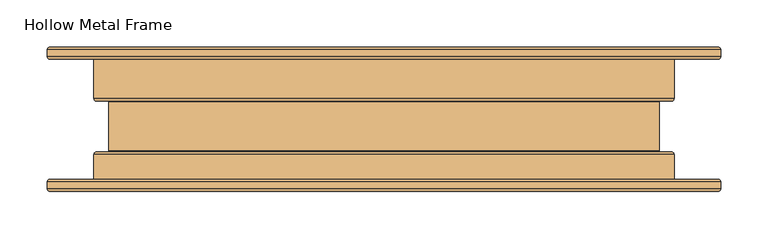
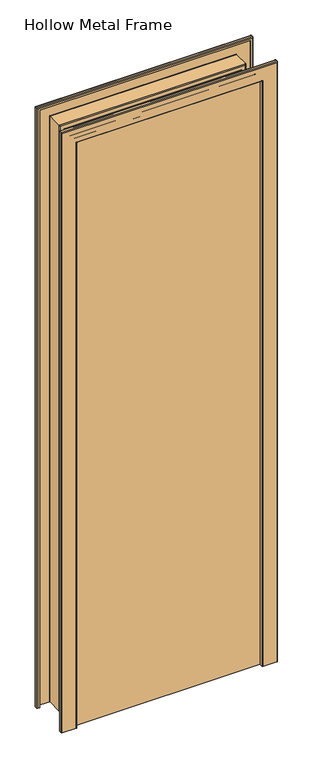
"""IFC4 building model written with IfcOpenShell, lengths in millimetres: door geometry, Hollow Metal Frame."""

from ifc_helpers import new_model, si_unit, frame, origin, origin_with_axes, place, context, project, spatial, polyline, circle_curve, ellipse_curve, outline, extrude, source, transform, mapped, element, save
from ifc_brep_helpers import plane_surface, cylinder_surface, revolved_surface, advanced_brep


def hollow_metal_frame_48c6d259(model_context):
    return source(origin(), model_context, "Body", "SolidModel", [
        advanced_brep(
        [(-353.02825, 63.5635, 0.0), (-355.6, 66.13525, 0.0), (-355.6, 73.66, 0.0), (-353.02825, 76.23175, 0.0), (-307.37175, 76.23175, 0.0), (-304.8, 73.66, 0.0), (-304.8, 21.68525, 0.0), (-303.784, 20.66925, 0.0), (-291.49675, 20.66925, 0.0), (-288.925, 18.0975, 0.0), (-288.925, -33.6931, 0.0), (-291.49675, -36.26485, 0.0), (-303.784, -36.26485, 0.0), (-304.8, -37.28085, 0.0), (-304.8, -73.5965, 0.0), (-307.37175, -76.16825, 0.0), (-353.02825, -76.16825, 0.0), (-355.6, -73.5965, 0.0), (-355.6, -66.07175, 0.0), (-353.02825, -63.5, 0.0), (-347.6625, -63.5, 0.0), (-347.6625, -65.05575, 0.0), (-353.02825, -65.05575, 0.0), (-354.04425, -66.07175, 0.0), (-354.04425, -73.5965, 0.0), (-353.02825, -74.6125, 0.0), (-307.37175, -74.6125, 0.0), (-306.35575, -73.5965, 0.0), (-306.35575, -37.28085, 0.0), (-303.784, -34.7091, 0.0), (-291.49675, -34.7091, 0.0), (-290.48075, -33.6931, 0.0), (-290.48075, 18.0975, 0.0), (-291.49675, 19.1135, 0.0), (-303.784, 19.1135, 0.0), (-306.35575, 21.68525, 0.0), (-306.35575, 73.66, 0.0), (-307.37175, 74.676, 0.0), (-353.02825, 74.676, 0.0), (-354.04425, 73.66, 0.0), (-354.04425, 66.13525, 0.0), (-353.02825, 65.11925, 0.0), (-347.6625, 65.11925, 0.0), (-347.6625, 63.5635, 0.0), (-353.02825, 63.5635, 2080.2282501), (-355.6, 66.13525, 2082.8000001), (-355.6, 73.66, 2082.8000001), (-353.02825, 76.23175, 2080.2282501), (353.02825, 76.23175, 2080.2282501), (353.02825, 76.23175, 0.0), (307.37175, 76.23175, 0.0), (307.37175, 76.23175, 2034.5717501), (-307.37175, 76.23175, 2034.5717501), (-304.8, 73.66, 2032.0000001), (-304.8, 21.68525, 2032.0000001), (-303.784, 20.66925, 2030.9840001), (303.784, 20.66925, 2030.9840001), (303.784, 20.66925, 0.0), (291.49675, 20.66925, 0.0), (291.49675, 20.66925, 2018.6967501), (-291.49675, 20.66925, 2018.6967501), (-288.925, 18.0975, 2016.1250001), (-288.925, -33.6931, 2016.1250001), (-291.49675, -36.26485, 2018.6967501), (291.49675, -36.26485, 2018.6967501), (291.49675, -36.26485, 0.0), (303.784, -36.26485, 0.0), (303.784, -36.26485, 2030.9840001), (-303.784, -36.26485, 2030.9840001), (-304.8, -37.28085, 2032.0000001), (-304.8, -73.5965, 2032.0000001), (-307.37175, -76.16825, 2034.5717501), (307.37175, -76.16825, 2034.5717501), (307.37175, -76.16825, 0.0), (353.02825, -76.16825, 0.0), (353.02825, -76.16825, 2080.2282501), (-353.02825, -76.16825, 2080.2282501), (-355.6, -73.5965, 2082.8000001), (-355.6, -66.07175, 2082.8000001), (-353.02825, -63.5, 2080.2282501), (353.02825, -63.5, 2080.2282501), (353.02825, -63.5, 0.0), (347.6625, -63.5, 0.0), (347.6625, -63.5, 2074.8625001), (-347.6625, -63.5, 2074.8625001), (-347.6625, -65.05575, 2074.8625001), (347.6625, -65.05575, 2074.8625001), (347.6625, -65.05575, 0.0), (353.02825, -65.05575, 0.0), (353.02825, -65.05575, 2080.2282501), (-353.02825, -65.05575, 2080.2282501), (-354.04425, -66.07175, 2081.2442501), (-354.04425, -73.5965, 2081.2442501), (-353.02825, -74.6125, 2080.2282501), (353.02825, -74.6125, 2080.2282501), (353.02825, -74.6125, 0.0), (307.37175, -74.6125, 0.0), (307.37175, -74.6125, 2034.5717501), (-307.37175, -74.6125, 2034.5717501), (-306.35575, -73.5965, 2033.5557501), (-306.35575, -37.28085, 2033.5557501), (-303.784, -34.7091, 2030.9840001), (303.784, -34.7091, 2030.9840001), (303.784, -34.7091, 0.0), (291.49675, -34.7091, 0.0), (291.49675, -34.7091, 2018.6967501), (-291.49675, -34.7091, 2018.6967501), (-290.48075, -33.6931, 2017.6807501), (-290.48075, 18.0975, 2017.6807501), (-291.49675, 19.1135, 2018.6967501), (291.49675, 19.1135, 2018.6967501), (291.49675, 19.1135, 0.0), (303.784, 19.1135, 0.0), (303.784, 19.1135, 2030.9840001), (-303.784, 19.1135, 2030.9840001), (-306.35575, 21.68525, 2033.5557501), (-306.35575, 73.66, 2033.5557501), (-307.37175, 74.676, 2034.5717501), (307.37175, 74.676, 2034.5717501), (307.37175, 74.676, 0.0), (353.02825, 74.676, 0.0), (353.02825, 74.676, 2080.2282501), (-353.02825, 74.676, 2080.2282501), (-354.04425, 73.66, 2081.2442501), (-354.04425, 66.13525, 2081.2442501), (-353.02825, 65.11925, 2080.2282501), (353.02825, 65.11925, 2080.2282501), (353.02825, 65.11925, 0.0), (347.6625, 65.11925, 0.0), (347.6625, 65.11925, 2074.8625001), (-347.6625, 65.11925, 2074.8625001), (-347.6625, 63.5635, 2074.8625001), (347.6625, 63.5635, 2074.8625001), (347.6625, 63.5635, 0.0), (353.02825, 63.5635, 0.0), (353.02825, 63.5635, 2080.2282501), (355.6, 66.13525, 2082.8000001), (355.6, 73.66, 2082.8000001), (304.8, 73.66, 2032.0000001), (304.8, 21.68525, 2032.0000001), (288.925, 18.0975, 2016.1250001), (288.925, -33.6931, 2016.1250001), (304.8, -37.28085, 2032.0000001), (304.8, -73.5965, 2032.0000001), (355.6, -73.5965, 2082.8000001), (355.6, -66.07175, 2082.8000001), (354.04425, -66.07175, 2081.2442501), (354.04425, -73.5965, 2081.2442501), (306.35575, -73.5965, 2033.5557501), (306.35575, -37.28085, 2033.5557501), (290.48075, -33.6931, 2017.6807501), (290.48075, 18.0975, 2017.6807501), (306.35575, 21.68525, 2033.5557501), (306.35575, 73.66, 2033.5557501), (354.04425, 73.66, 2081.2442501), (354.04425, 66.13525, 2081.2442501), (354.04425, 66.13525, 0.0), (354.04425, 73.66, 0.0), (306.35575, 73.66, 0.0), (306.35575, 21.68525, 0.0), (290.48075, 18.0975, 0.0), (290.48075, -33.6931, 0.0), (306.35575, -37.28085, 0.0), (306.35575, -73.5965, 0.0), (354.04425, -73.5965, 0.0), (354.04425, -66.07175, 0.0), (355.6, -66.07175, 0.0), (355.6, -73.5965, 0.0), (304.8, -73.5965, 0.0), (304.8, -37.28085, 0.0), (288.925, -33.6931, 0.0), (288.925, 18.0975, 0.0), (304.8, 21.68525, 0.0), (304.8, 73.66, 0.0), (355.6, 73.66, 0.0), (355.6, 66.13525, 0.0)],
        [
            (0, 1, circle_curve(frame((-353.02825, 66.13525, 0.0), z_axis=(0.0, 0.0, -1.0), x_axis=(0.0, -1.0, 0.0)), 2.57175)),
            (1, 2),
            (2, 3, circle_curve(frame((-353.02825, 73.66, 0.0), z_axis=(0.0, 0.0, -1.0), x_axis=(0.0, -1.0, 0.0)), 2.57175)),
            (3, 4),
            (4, 5, circle_curve(frame((-307.37175, 73.66, 0.0), z_axis=(0.0, 0.0, -1.0), x_axis=(0.0, -1.0, 0.0)), 2.57175)),
            (5, 6),
            (6, 7, circle_curve(frame((-303.784, 21.68525, 0.0), z_axis=(0.0, 0.0, 1.0), x_axis=(0.0, -1.0, 0.0)), 1.016)),
            (7, 8),
            (8, 9, circle_curve(frame((-291.49675, 18.0975, 0.0), z_axis=(0.0, 0.0, -1.0), x_axis=(0.0, -1.0, 0.0)), 2.57175)),
            (9, 10),
            (10, 11, circle_curve(frame((-291.49675, -33.6931, 0.0), z_axis=(0.0, 0.0, -1.0), x_axis=(0.0, -1.0, 0.0)), 2.57175)),
            (11, 12),
            (12, 13, circle_curve(frame((-303.784, -37.28085, 0.0), z_axis=(0.0, 0.0, 1.0), x_axis=(0.0, -1.0, 0.0)), 1.016)),
            (13, 14),
            (14, 15, circle_curve(frame((-307.37175, -73.5965, 0.0), z_axis=(0.0, 0.0, -1.0), x_axis=(0.0, -1.0, 0.0)), 2.57175)),
            (15, 16),
            (16, 17, circle_curve(frame((-353.02825, -73.5965, 0.0), z_axis=(0.0, 0.0, -1.0), x_axis=(0.0, -1.0, 0.0)), 2.57175)),
            (17, 18),
            (18, 19, circle_curve(frame((-353.02825, -66.07175, 0.0), z_axis=(0.0, 0.0, -1.0), x_axis=(0.0, -1.0, 0.0)), 2.57175)),
            (19, 20),
            (20, 21),
            (21, 22),
            (22, 23, circle_curve(frame((-353.02825, -66.07175, 0.0), z_axis=(0.0, 0.0, 1.0), x_axis=(0.0, -1.0, 0.0)), 1.016)),
            (23, 24),
            (24, 25, circle_curve(frame((-353.02825, -73.5965, 0.0), z_axis=(0.0, 0.0, 1.0), x_axis=(0.0, -1.0, 0.0)), 1.016)),
            (25, 26),
            (26, 27, circle_curve(frame((-307.37175, -73.5965, 0.0), z_axis=(0.0, 0.0, 1.0), x_axis=(0.0, -1.0, 0.0)), 1.016)),
            (27, 28),
            (28, 29, circle_curve(frame((-303.784, -37.28085, 0.0), z_axis=(0.0, 0.0, -1.0), x_axis=(0.0, -1.0, 0.0)), 2.57175)),
            (29, 30),
            (30, 31, circle_curve(frame((-291.49675, -33.6931, 0.0), z_axis=(0.0, 0.0, 1.0), x_axis=(0.0, -1.0, 0.0)), 1.016)),
            (31, 32),
            (32, 33, circle_curve(frame((-291.49675, 18.0975, 0.0), z_axis=(0.0, 0.0, 1.0), x_axis=(0.0, -1.0, 0.0)), 1.016)),
            (33, 34),
            (34, 35, circle_curve(frame((-303.784, 21.68525, 0.0), z_axis=(0.0, 0.0, -1.0), x_axis=(0.0, -1.0, 0.0)), 2.57175)),
            (35, 36),
            (36, 37, circle_curve(frame((-307.37175, 73.66, 0.0), z_axis=(0.0, 0.0, 1.0), x_axis=(0.0, -1.0, 0.0)), 1.016)),
            (37, 38),
            (38, 39, circle_curve(frame((-353.02825, 73.66, 0.0), z_axis=(0.0, 0.0, 1.0), x_axis=(0.0, -1.0, 0.0)), 1.016)),
            (39, 40),
            (40, 41, circle_curve(frame((-353.02825, 66.13525, 0.0), z_axis=(0.0, 0.0, 1.0), x_axis=(0.0, -1.0, 0.0)), 1.016)),
            (41, 42),
            (42, 43),
            (43, 0),
            (0, 44),
            (44, 45, ellipse_curve(frame((-353.02825, 66.13525, 2080.2282501), z_axis=(-0.7071067811865475, 0.0, -0.7071067811865475), x_axis=(0.7071067811865474, 0.0, -0.7071067811865476)), 3.6370037, 2.57175)),
            (45, 1),
            (45, 46),
            (46, 2),
            (46, 47, ellipse_curve(frame((-353.02825, 73.66, 2080.2282501), z_axis=(-0.7071067811865475, 0.0, -0.7071067811865475), x_axis=(0.7071067811865474, 0.0, -0.7071067811865476)), 3.6370037, 2.57175)),
            (47, 3),
            (47, 48),
            (48, 49),
            (49, 50),
            (50, 51),
            (51, 52),
            (52, 4),
            (52, 53, ellipse_curve(frame((-307.37175, 73.66, 2034.5717501), z_axis=(-0.7071067811865475, 0.0, -0.7071067811865475), x_axis=(0.7071067811865474, 0.0, -0.7071067811865476)), 3.6370037, 2.57175)),
            (53, 5),
            (53, 54),
            (54, 6),
            (54, 55, ellipse_curve(frame((-303.784, 21.68525, 2030.9840001), z_axis=(0.7071067811865475, 0.0, 0.7071067811865475), x_axis=(-0.7071067811865474, 0.0, 0.7071067811865476)), 1.436841, 1.016)),
            (55, 7),
            (55, 56),
            (56, 57),
            (57, 58),
            (58, 59),
            (59, 60),
            (60, 8),
            (60, 61, ellipse_curve(frame((-291.49675, 18.0975, 2018.6967501), z_axis=(-0.7071067811865475, 0.0, -0.7071067811865475), x_axis=(0.7071067811865474, 0.0, -0.7071067811865476)), 3.6370037, 2.57175)),
            (61, 9),
            (61, 62),
            (62, 10),
            (62, 63, ellipse_curve(frame((-291.49675, -33.6931, 2018.6967501), z_axis=(-0.7071067811865475, 0.0, -0.7071067811865475), x_axis=(0.7071067811865474, 0.0, -0.7071067811865476)), 3.6370037, 2.57175)),
            (63, 11),
            (63, 64),
            (64, 65),
            (65, 66),
            (66, 67),
            (67, 68),
            (68, 12),
            (68, 69, ellipse_curve(frame((-303.784, -37.28085, 2030.9840001), z_axis=(0.7071067811865475, 0.0, 0.7071067811865475), x_axis=(-0.7071067811865474, 0.0, 0.7071067811865476)), 1.436841, 1.016)),
            (69, 13),
            (69, 70),
            (70, 14),
            (70, 71, ellipse_curve(frame((-307.37175, -73.5965, 2034.5717501), z_axis=(-0.7071067811865475, 0.0, -0.7071067811865475), x_axis=(0.7071067811865474, 0.0, -0.7071067811865476)), 3.6370037, 2.57175)),
            (71, 15),
            (71, 72),
            (72, 73),
            (73, 74),
            (74, 75),
            (75, 76),
            (76, 16),
            (76, 77, ellipse_curve(frame((-353.02825, -73.5965, 2080.2282501), z_axis=(-0.7071067811865475, 0.0, -0.7071067811865475), x_axis=(0.7071067811865474, 0.0, -0.7071067811865476)), 3.6370037, 2.57175)),
            (77, 17),
            (77, 78),
            (78, 18),
            (78, 79, ellipse_curve(frame((-353.02825, -66.07175, 2080.2282501), z_axis=(-0.7071067811865475, 0.0, -0.7071067811865475), x_axis=(0.7071067811865474, 0.0, -0.7071067811865476)), 3.6370037, 2.57175)),
            (79, 19),
            (79, 80),
            (80, 81),
            (81, 82),
            (82, 83),
            (83, 84),
            (84, 20),
            (84, 85),
            (85, 21),
            (85, 86),
            (86, 87),
            (87, 88),
            (88, 89),
            (89, 90),
            (90, 22),
            (90, 91, ellipse_curve(frame((-353.02825, -66.07175, 2080.2282501), z_axis=(0.7071067811865475, 0.0, 0.7071067811865475), x_axis=(-0.7071067811865474, 0.0, 0.7071067811865476)), 1.436841, 1.016)),
            (91, 23),
            (91, 92),
            (92, 24),
            (92, 93, ellipse_curve(frame((-353.02825, -73.5965, 2080.2282501), z_axis=(0.7071067811865475, 0.0, 0.7071067811865475), x_axis=(-0.7071067811865474, 0.0, 0.7071067811865476)), 1.436841, 1.016)),
            (93, 25),
            (93, 94),
            (94, 95),
            (95, 96),
            (96, 97),
            (97, 98),
            (98, 26),
            (98, 99, ellipse_curve(frame((-307.37175, -73.5965, 2034.5717501), z_axis=(0.7071067811865475, 0.0, 0.7071067811865475), x_axis=(-0.7071067811865474, 0.0, 0.7071067811865476)), 1.436841, 1.016)),
            (99, 27),
            (99, 100),
            (100, 28),
            (100, 101, ellipse_curve(frame((-303.784, -37.28085, 2030.9840001), z_axis=(-0.7071067811865475, 0.0, -0.7071067811865475), x_axis=(0.7071067811865474, 0.0, -0.7071067811865476)), 3.6370037, 2.57175)),
            (101, 29),
            (101, 102),
            (102, 103),
            (103, 104),
            (104, 105),
            (105, 106),
            (106, 30),
            (106, 107, ellipse_curve(frame((-291.49675, -33.6931, 2018.6967501), z_axis=(0.7071067811865475, 0.0, 0.7071067811865475), x_axis=(-0.7071067811865474, 0.0, 0.7071067811865476)), 1.436841, 1.016)),
            (107, 31),
            (107, 108),
            (108, 32),
            (108, 109, ellipse_curve(frame((-291.49675, 18.0975, 2018.6967501), z_axis=(0.7071067811865475, 0.0, 0.7071067811865475), x_axis=(-0.7071067811865474, 0.0, 0.7071067811865476)), 1.436841, 1.016)),
            (109, 33),
            (109, 110),
            (110, 111),
            (111, 112),
            (112, 113),
            (113, 114),
            (114, 34),
            (114, 115, ellipse_curve(frame((-303.784, 21.68525, 2030.9840001), z_axis=(-0.7071067811865475, 0.0, -0.7071067811865475), x_axis=(0.7071067811865474, 0.0, -0.7071067811865476)), 3.6370037, 2.57175)),
            (115, 35),
            (115, 116),
            (116, 36),
            (116, 117, ellipse_curve(frame((-307.37175, 73.66, 2034.5717501), z_axis=(0.7071067811865475, 0.0, 0.7071067811865475), x_axis=(-0.7071067811865474, 0.0, 0.7071067811865476)), 1.436841, 1.016)),
            (117, 37),
            (117, 118),
            (118, 119),
            (119, 120),
            (120, 121),
            (121, 122),
            (122, 38),
            (122, 123, ellipse_curve(frame((-353.02825, 73.66, 2080.2282501), z_axis=(0.7071067811865475, 0.0, 0.7071067811865475), x_axis=(-0.7071067811865474, 0.0, 0.7071067811865476)), 1.436841, 1.016)),
            (123, 39),
            (123, 124),
            (124, 40),
            (124, 125, ellipse_curve(frame((-353.02825, 66.13525, 2080.2282501), z_axis=(0.7071067811865475, 0.0, 0.7071067811865475), x_axis=(-0.7071067811865474, 0.0, 0.7071067811865476)), 1.436841, 1.016)),
            (125, 41),
            (125, 126),
            (126, 127),
            (127, 128),
            (128, 129),
            (129, 130),
            (130, 42),
            (130, 131),
            (131, 43),
            (131, 132),
            (132, 133),
            (133, 134),
            (134, 135),
            (135, 44),
            (135, 136, ellipse_curve(frame((353.02825, 66.13525, 2080.2282501), z_axis=(-0.7071067811865475, 0.0, 0.7071067811865475), x_axis=(-0.7071067811865476, 0.0, -0.7071067811865474)), 3.6370037, 2.57175)),
            (136, 45),
            (136, 137),
            (137, 46),
            (137, 48, ellipse_curve(frame((353.02825, 73.66, 2080.2282501), z_axis=(-0.7071067811865475, 0.0, 0.7071067811865475), x_axis=(-0.7071067811865476, 0.0, -0.7071067811865474)), 3.6370037, 2.57175)),
            (51, 138, ellipse_curve(frame((307.37175, 73.66, 2034.5717501), z_axis=(-0.7071067811865475, 0.0, 0.7071067811865475), x_axis=(-0.7071067811865476, 0.0, -0.7071067811865474)), 3.6370037, 2.57175)),
            (138, 53),
            (138, 139),
            (139, 54),
            (139, 56, ellipse_curve(frame((303.784, 21.68525, 2030.9840001), z_axis=(0.7071067811865475, 0.0, -0.7071067811865475), x_axis=(0.7071067811865476, 0.0, 0.7071067811865474)), 1.436841, 1.016)),
            (59, 140, ellipse_curve(frame((291.49675, 18.0975, 2018.6967501), z_axis=(-0.7071067811865475, 0.0, 0.7071067811865475), x_axis=(-0.7071067811865476, 0.0, -0.7071067811865474)), 3.6370037, 2.57175)),
            (140, 61),
            (140, 141),
            (141, 62),
            (141, 64, ellipse_curve(frame((291.49675, -33.6931, 2018.6967501), z_axis=(-0.7071067811865475, 0.0, 0.7071067811865475), x_axis=(-0.7071067811865476, 0.0, -0.7071067811865474)), 3.6370037, 2.57175)),
            (67, 142, ellipse_curve(frame((303.784, -37.28085, 2030.9840001), z_axis=(0.7071067811865475, 0.0, -0.7071067811865475), x_axis=(0.7071067811865476, 0.0, 0.7071067811865474)), 1.436841, 1.016)),
            (142, 69),
            (142, 143),
            (143, 70),
            (143, 72, ellipse_curve(frame((307.37175, -73.5965, 2034.5717501), z_axis=(-0.7071067811865475, 0.0, 0.7071067811865475), x_axis=(-0.7071067811865476, 0.0, -0.7071067811865474)), 3.6370037, 2.57175)),
            (75, 144, ellipse_curve(frame((353.02825, -73.5965, 2080.2282501), z_axis=(-0.7071067811865475, 0.0, 0.7071067811865475), x_axis=(-0.7071067811865476, 0.0, -0.7071067811865474)), 3.6370037, 2.57175)),
            (144, 77),
            (144, 145),
            (145, 78),
            (145, 80, ellipse_curve(frame((353.02825, -66.07175, 2080.2282501), z_axis=(-0.7071067811865475, 0.0, 0.7071067811865475), x_axis=(-0.7071067811865476, 0.0, -0.7071067811865474)), 3.6370037, 2.57175)),
            (83, 86),
            (89, 146, ellipse_curve(frame((353.02825, -66.07175, 2080.2282501), z_axis=(0.7071067811865475, 0.0, -0.7071067811865475), x_axis=(0.7071067811865476, 0.0, 0.7071067811865474)), 1.436841, 1.016)),
            (146, 91),
            (146, 147),
            (147, 92),
            (147, 94, ellipse_curve(frame((353.02825, -73.5965, 2080.2282501), z_axis=(0.7071067811865475, 0.0, -0.7071067811865475), x_axis=(0.7071067811865476, 0.0, 0.7071067811865474)), 1.436841, 1.016)),
            (97, 148, ellipse_curve(frame((307.37175, -73.5965, 2034.5717501), z_axis=(0.7071067811865475, 0.0, -0.7071067811865475), x_axis=(0.7071067811865476, 0.0, 0.7071067811865474)), 1.436841, 1.016)),
            (148, 99),
            (148, 149),
            (149, 100),
            (149, 102, ellipse_curve(frame((303.784, -37.28085, 2030.9840001), z_axis=(-0.7071067811865475, 0.0, 0.7071067811865475), x_axis=(-0.7071067811865476, 0.0, -0.7071067811865474)), 3.6370037, 2.57175)),
            (105, 150, ellipse_curve(frame((291.49675, -33.6931, 2018.6967501), z_axis=(0.7071067811865475, 0.0, -0.7071067811865475), x_axis=(0.7071067811865476, 0.0, 0.7071067811865474)), 1.436841, 1.016)),
            (150, 107),
            (150, 151),
            (151, 108),
            (151, 110, ellipse_curve(frame((291.49675, 18.0975, 2018.6967501), z_axis=(0.7071067811865475, 0.0, -0.7071067811865475), x_axis=(0.7071067811865476, 0.0, 0.7071067811865474)), 1.436841, 1.016)),
            (113, 152, ellipse_curve(frame((303.784, 21.68525, 2030.9840001), z_axis=(-0.7071067811865475, 0.0, 0.7071067811865475), x_axis=(-0.7071067811865476, 0.0, -0.7071067811865474)), 3.6370037, 2.57175)),
            (152, 115),
            (152, 153),
            (153, 116),
            (153, 118, ellipse_curve(frame((307.37175, 73.66, 2034.5717501), z_axis=(0.7071067811865475, 0.0, -0.7071067811865475), x_axis=(0.7071067811865476, 0.0, 0.7071067811865474)), 1.436841, 1.016)),
            (121, 154, ellipse_curve(frame((353.02825, 73.66, 2080.2282501), z_axis=(0.7071067811865475, 0.0, -0.7071067811865475), x_axis=(0.7071067811865476, 0.0, 0.7071067811865474)), 1.436841, 1.016)),
            (154, 123),
            (154, 155),
            (155, 124),
            (155, 126, ellipse_curve(frame((353.02825, 66.13525, 2080.2282501), z_axis=(0.7071067811865475, 0.0, -0.7071067811865475), x_axis=(0.7071067811865476, 0.0, 0.7071067811865474)), 1.436841, 1.016)),
            (129, 132),
            (133, 128),
            (127, 156, circle_curve(frame((353.02825, 66.13525, 0.0), z_axis=(0.0, 0.0, 1.0), x_axis=(0.0, -1.0, 0.0)), 1.016)),
            (156, 157),
            (157, 120, circle_curve(frame((353.02825, 73.66, 0.0), z_axis=(0.0, 0.0, 1.0), x_axis=(0.0, -1.0, 0.0)), 1.016)),
            (119, 158, circle_curve(frame((307.37175, 73.66, 0.0), z_axis=(0.0, 0.0, 1.0), x_axis=(0.0, -1.0, 0.0)), 1.016)),
            (158, 159),
            (159, 112, circle_curve(frame((303.784, 21.68525, 0.0), z_axis=(0.0, 0.0, -1.0), x_axis=(0.0, -1.0, 0.0)), 2.57175)),
            (111, 160, circle_curve(frame((291.49675, 18.0975, 0.0), z_axis=(0.0, 0.0, 1.0), x_axis=(0.0, -1.0, 0.0)), 1.016)),
            (160, 161),
            (161, 104, circle_curve(frame((291.49675, -33.6931, 0.0), z_axis=(0.0, 0.0, 1.0), x_axis=(0.0, -1.0, 0.0)), 1.016)),
            (103, 162, circle_curve(frame((303.784, -37.28085, 0.0), z_axis=(0.0, 0.0, -1.0), x_axis=(0.0, -1.0, 0.0)), 2.57175)),
            (162, 163),
            (163, 96, circle_curve(frame((307.37175, -73.5965, 0.0), z_axis=(0.0, 0.0, 1.0), x_axis=(0.0, -1.0, 0.0)), 1.016)),
            (95, 164, circle_curve(frame((353.02825, -73.5965, 0.0), z_axis=(0.0, 0.0, 1.0), x_axis=(0.0, -1.0, 0.0)), 1.016)),
            (164, 165),
            (165, 88, circle_curve(frame((353.02825, -66.07175, 0.0), z_axis=(0.0, 0.0, 1.0), x_axis=(0.0, -1.0, 0.0)), 1.016)),
            (87, 82),
            (81, 166, circle_curve(frame((353.02825, -66.07175, 0.0), z_axis=(0.0, 0.0, -1.0), x_axis=(0.0, -1.0, 0.0)), 2.57175)),
            (166, 167),
            (167, 74, circle_curve(frame((353.02825, -73.5965, 0.0), z_axis=(0.0, 0.0, -1.0), x_axis=(0.0, -1.0, 0.0)), 2.57175)),
            (73, 168, circle_curve(frame((307.37175, -73.5965, 0.0), z_axis=(0.0, 0.0, -1.0), x_axis=(0.0, -1.0, 0.0)), 2.57175)),
            (168, 169),
            (169, 66, circle_curve(frame((303.784, -37.28085, 0.0), z_axis=(0.0, 0.0, 1.0), x_axis=(0.0, -1.0, 0.0)), 1.016)),
            (65, 170, circle_curve(frame((291.49675, -33.6931, 0.0), z_axis=(0.0, 0.0, -1.0), x_axis=(0.0, -1.0, 0.0)), 2.57175)),
            (170, 171),
            (171, 58, circle_curve(frame((291.49675, 18.0975, 0.0), z_axis=(0.0, 0.0, -1.0), x_axis=(0.0, -1.0, 0.0)), 2.57175)),
            (57, 172, circle_curve(frame((303.784, 21.68525, 0.0), z_axis=(0.0, 0.0, 1.0), x_axis=(0.0, -1.0, 0.0)), 1.016)),
            (172, 173),
            (173, 50, circle_curve(frame((307.37175, 73.66, 0.0), z_axis=(0.0, 0.0, -1.0), x_axis=(0.0, -1.0, 0.0)), 2.57175)),
            (49, 174, circle_curve(frame((353.02825, 73.66, 0.0), z_axis=(0.0, 0.0, -1.0), x_axis=(0.0, -1.0, 0.0)), 2.57175)),
            (174, 175),
            (175, 134, circle_curve(frame((353.02825, 66.13525, 0.0), z_axis=(0.0, 0.0, -1.0), x_axis=(0.0, -1.0, 0.0)), 2.57175)),
            (175, 136),
            (174, 137),
            (173, 138),
            (172, 139),
            (171, 140),
            (170, 141),
            (169, 142),
            (168, 143),
            (167, 144),
            (166, 145),
            (165, 146),
            (164, 147),
            (163, 148),
            (162, 149),
            (161, 150),
            (160, 151),
            (159, 152),
            (158, 153),
            (157, 154),
            (156, 155),
        ],
        [
            plane_surface(frame((-315.9125, -63.5, 0.0), z_axis=(0.0, 0.0, -1.0), x_axis=(1.0, 0.0, 0.0))),
            cylinder_surface(frame((-353.02825, 66.13525, 0.0), z_axis=(0.0, 0.0, -1.0), x_axis=(0.0, -1.0, 0.0)), 2.57175),
            plane_surface(frame((-355.6, 66.13525, 0.0), z_axis=(-1.0, 0.0, 0.0), x_axis=(0.0, 0.0, 1.0))),
            cylinder_surface(frame((-353.02825, 73.66, 0.0), z_axis=(0.0, 0.0, -1.0), x_axis=(0.0, -1.0, 0.0)), 2.57175),
            plane_surface(frame((-353.02825, 76.23175, 0.0), z_axis=(0.0, 1.0, 0.0), x_axis=(0.0, 0.0, 1.0))),
            cylinder_surface(frame((-307.37175, 73.66, 0.0), z_axis=(0.0, 0.0, -1.0), x_axis=(0.0, -1.0, 0.0)), 2.57175),
            plane_surface(frame((-304.8, 73.66, 0.0), z_axis=(1.0, 0.0, 0.0), x_axis=(0.0, 0.0, 1.0))),
            revolved_surface(polyline([(-303.784, 20.669249999999998, 2032.0000001145868), (-303.784, 20.669249999999998, 0.0)]), (-303.784, 21.68525, 0.0), (0.0, 0.0, 1.0)),
            plane_surface(frame((-303.784, 20.66925, 0.0), z_axis=(0.0, 1.0, 0.0), x_axis=(0.0, 0.0, 1.0))),
            cylinder_surface(frame((-291.49675, 18.0975, 0.0), z_axis=(0.0, 0.0, -1.0), x_axis=(0.0, -1.0, 0.0)), 2.57175),
            plane_surface(frame((-288.925, 18.0975, 0.0), z_axis=(1.0, 0.0, 0.0), x_axis=(0.0, 0.0, 1.0))),
            cylinder_surface(frame((-291.49675, -33.6931, 0.0), z_axis=(0.0, 0.0, -1.0), x_axis=(0.0, -1.0, 0.0)), 2.57175),
            plane_surface(frame((-291.49675, -36.26485, 0.0), z_axis=(0.0, -1.0, 0.0), x_axis=(0.0, 0.0, 1.0))),
            revolved_surface(polyline([(-303.784, -38.29685, 2032.0000001145868), (-303.784, -38.29685, 0.0)]), (-303.784, -37.28085, 0.0), (0.0, 0.0, 1.0)),
            plane_surface(frame((-304.8, -37.28085, 0.0), z_axis=(1.0, 0.0, 0.0), x_axis=(0.0, 0.0, 1.0))),
            cylinder_surface(frame((-307.37175, -73.5965, 0.0), z_axis=(0.0, 0.0, -1.0), x_axis=(0.0, -1.0, 0.0)), 2.57175),
            plane_surface(frame((-307.37175, -76.16825, 0.0), z_axis=(0.0, -1.0, 0.0), x_axis=(0.0, 0.0, 1.0))),
            cylinder_surface(frame((-353.02825, -73.5965, 0.0), z_axis=(0.0, 0.0, -1.0), x_axis=(0.0, -1.0, 0.0)), 2.57175),
            plane_surface(frame((-355.6, -73.5965, 0.0), z_axis=(-1.0, 0.0, 0.0), x_axis=(0.0, 0.0, 1.0))),
            cylinder_surface(frame((-353.02825, -66.07175, 0.0), z_axis=(0.0, 0.0, -1.0), x_axis=(0.0, -1.0, 0.0)), 2.57175),
            plane_surface(frame((-353.02825, -63.5, 0.0), z_axis=(0.0, 1.0, 0.0), x_axis=(0.0, 0.0, 1.0))),
            plane_surface(frame((-347.6625, -63.5, 0.0), z_axis=(1.0, 0.0, 0.0), x_axis=(0.0, 0.0, 1.0))),
            plane_surface(frame((-347.6625, -65.05575, 0.0), z_axis=(0.0, -1.0, 0.0), x_axis=(0.0, 0.0, 1.0))),
            revolved_surface(polyline([(-353.02825, -67.08775, 2081.244250114587), (-353.02825, -67.08775, 0.0)]), (-353.02825, -66.07175, 0.0), (0.0, 0.0, 1.0)),
            plane_surface(frame((-354.04425, -66.07175, 0.0), z_axis=(1.0, 0.0, 0.0), x_axis=(0.0, 0.0, 1.0))),
            revolved_surface(polyline([(-353.02825, -74.61250000000001, 2081.244250114587), (-353.02825, -74.61250000000001, 0.0)]), (-353.02825, -73.5965, 0.0), (0.0, 0.0, 1.0)),
            plane_surface(frame((-353.02825, -74.6125, 0.0), z_axis=(0.0, 1.0, 0.0), x_axis=(0.0, 0.0, 1.0))),
            revolved_surface(polyline([(-307.37175, -74.61250000000001, 2035.5877501145867), (-307.37175, -74.61250000000001, 0.0)]), (-307.37175, -73.5965, 0.0), (0.0, 0.0, 1.0)),
            plane_surface(frame((-306.35575, -73.5965, 0.0), z_axis=(-1.0, 0.0, 0.0), x_axis=(0.0, 0.0, 1.0))),
            cylinder_surface(frame((-303.784, -37.28085, 0.0), z_axis=(0.0, 0.0, -1.0), x_axis=(0.0, -1.0, 0.0)), 2.57175),
            plane_surface(frame((-303.784, -34.7091, 0.0), z_axis=(0.0, 1.0, 0.0), x_axis=(0.0, 0.0, 1.0))),
            revolved_surface(polyline([(-291.49675, -34.7091, 2019.7127501145867), (-291.49675, -34.7091, 0.0)]), (-291.49675, -33.6931, 0.0), (0.0, 0.0, 1.0)),
            plane_surface(frame((-290.48075, -33.6931, 0.0), z_axis=(-1.0, 0.0, 0.0), x_axis=(0.0, 0.0, 1.0))),
            revolved_surface(polyline([(-291.49675, 17.0815, 2019.7127501145867), (-291.49675, 17.0815, 0.0)]), (-291.49675, 18.0975, 0.0), (0.0, 0.0, 1.0)),
            plane_surface(frame((-291.49675, 19.1135, 0.0), z_axis=(0.0, -1.0, 0.0), x_axis=(0.0, 0.0, 1.0))),
            cylinder_surface(frame((-303.784, 21.68525, 0.0), z_axis=(0.0, 0.0, -1.0), x_axis=(0.0, -1.0, 0.0)), 2.57175),
            plane_surface(frame((-306.35575, 21.68525, 0.0), z_axis=(-1.0, 0.0, 0.0), x_axis=(0.0, 0.0, 1.0))),
            revolved_surface(polyline([(-307.37175, 72.64399999999999, 2035.5877501145867), (-307.37175, 72.64399999999999, 0.0)]), (-307.37175, 73.66, 0.0), (0.0, 0.0, 1.0)),
            plane_surface(frame((-307.37175, 74.676, 0.0), z_axis=(0.0, -1.0, 0.0), x_axis=(0.0, 0.0, 1.0))),
            revolved_surface(polyline([(-353.02825, 72.64399999999999, 2081.244250114587), (-353.02825, 72.64399999999999, 0.0)]), (-353.02825, 73.66, 0.0), (0.0, 0.0, 1.0)),
            plane_surface(frame((-354.04425, 73.66, 0.0), z_axis=(1.0, 0.0, 0.0), x_axis=(0.0, 0.0, 1.0))),
            revolved_surface(polyline([(-353.02825, 65.11925, 2081.244250114587), (-353.02825, 65.11925, 0.0)]), (-353.02825, 66.13525, 0.0), (0.0, 0.0, 1.0)),
            plane_surface(frame((-353.02825, 65.11925, 0.0), z_axis=(0.0, 1.0, 0.0), x_axis=(0.0, 0.0, 1.0))),
            plane_surface(frame((-347.6625, 65.11925, 0.0), z_axis=(1.0, 0.0, 0.0), x_axis=(0.0, 0.0, 1.0))),
            plane_surface(frame((-347.6625, 63.5635, 0.0), z_axis=(0.0, -1.0, 0.0), x_axis=(0.0, 0.0, 1.0))),
            cylinder_surface(frame((-315.9125, 66.13525, 2080.2282501), z_axis=(-1.0, 0.0, 0.0), x_axis=(0.0, -1.0, 0.0)), 2.57175),
            plane_surface(frame((-355.6, 66.13525, 2082.8000001), z_axis=(0.0, 0.0, 1.0), x_axis=(1.0, 0.0, 0.0))),
            cylinder_surface(frame((-315.9125, 73.66, 2080.2282501), z_axis=(-1.0, 0.0, 0.0), x_axis=(0.0, -1.0, 0.0)), 2.57175),
            cylinder_surface(frame((-315.9125, 73.66, 2034.5717501), z_axis=(-1.0, 0.0, 0.0), x_axis=(0.0, -1.0, 0.0)), 2.57175),
            plane_surface(frame((-304.8, 73.66, 2032.0000001), z_axis=(0.0, 0.0, -1.0), x_axis=(1.0, 0.0, 0.0))),
            revolved_surface(polyline([(304.8000000145869, 20.669249999999998, 2030.9840001), (-304.80000001458683, 20.669249999999998, 2030.9840001)]), (-315.9125, 21.68525, 2030.9840001), (1.0, 0.0, 0.0)),
            cylinder_surface(frame((-315.9125, 18.0975, 2018.6967501), z_axis=(-1.0, 0.0, 0.0), x_axis=(0.0, -1.0, 0.0)), 2.57175),
            plane_surface(frame((-288.925, 18.0975, 2016.1250001), z_axis=(0.0, 0.0, -1.0), x_axis=(1.0, 0.0, 0.0))),
            cylinder_surface(frame((-315.9125, -33.6931, 2018.6967501), z_axis=(-1.0, 0.0, 0.0), x_axis=(0.0, -1.0, 0.0)), 2.57175),
            revolved_surface(polyline([(304.8000000145869, -38.29685, 2030.9840001), (-304.80000001458683, -38.29685, 2030.9840001)]), (-315.9125, -37.28085, 2030.9840001), (1.0, 0.0, 0.0)),
            plane_surface(frame((-304.8, -37.28085, 2032.0000001), z_axis=(0.0, 0.0, -1.0), x_axis=(1.0, 0.0, 0.0))),
            cylinder_surface(frame((-315.9125, -73.5965, 2034.5717501), z_axis=(-1.0, 0.0, 0.0), x_axis=(0.0, -1.0, 0.0)), 2.57175),
            cylinder_surface(frame((-315.9125, -73.5965, 2080.2282501), z_axis=(-1.0, 0.0, 0.0), x_axis=(0.0, -1.0, 0.0)), 2.57175),
            plane_surface(frame((-355.6, -73.5965, 2082.8000001), z_axis=(0.0, 0.0, 1.0), x_axis=(1.0, 0.0, 0.0))),
            cylinder_surface(frame((-315.9125, -66.07175, 2080.2282501), z_axis=(-1.0, 0.0, 0.0), x_axis=(0.0, -1.0, 0.0)), 2.57175),
            plane_surface(frame((-347.6625, -63.5, 2074.8625001), z_axis=(0.0, 0.0, -1.0), x_axis=(1.0, 0.0, 0.0))),
            revolved_surface(polyline([(354.04425001458685, -67.08775, 2080.2282501), (-354.04425001458685, -67.08775, 2080.2282501)]), (-315.9125, -66.07175, 2080.2282501), (1.0, 0.0, 0.0)),
            plane_surface(frame((-354.04425, -66.07175, 2081.2442501), z_axis=(0.0, 0.0, -1.0), x_axis=(1.0, 0.0, 0.0))),
            revolved_surface(polyline([(354.04425001458685, -74.61250000000001, 2080.2282501), (-354.04425001458685, -74.61250000000001, 2080.2282501)]), (-315.9125, -73.5965, 2080.2282501), (1.0, 0.0, 0.0)),
            revolved_surface(polyline([(308.3877500145869, -74.61250000000001, 2034.5717501), (-308.38775001458686, -74.61250000000001, 2034.5717501)]), (-315.9125, -73.5965, 2034.5717501), (1.0, 0.0, 0.0)),
            plane_surface(frame((-306.35575, -73.5965, 2033.5557501), z_axis=(0.0, 0.0, 1.0), x_axis=(1.0, 0.0, 0.0))),
            cylinder_surface(frame((-315.9125, -37.28085, 2030.9840001), z_axis=(-1.0, 0.0, 0.0), x_axis=(0.0, -1.0, 0.0)), 2.57175),
            revolved_surface(polyline([(292.5127500145869, -34.7091, 2018.6967501), (-292.51275001458686, -34.7091, 2018.6967501)]), (-315.9125, -33.6931, 2018.6967501), (1.0, 0.0, 0.0)),
            plane_surface(frame((-290.48075, -33.6931, 2017.6807501), z_axis=(0.0, 0.0, 1.0), x_axis=(1.0, 0.0, 0.0))),
            revolved_surface(polyline([(292.5127500145869, 17.0815, 2018.6967501), (-292.51275001458686, 17.0815, 2018.6967501)]), (-315.9125, 18.0975, 2018.6967501), (1.0, 0.0, 0.0)),
            cylinder_surface(frame((-315.9125, 21.68525, 2030.9840001), z_axis=(-1.0, 0.0, 0.0), x_axis=(0.0, -1.0, 0.0)), 2.57175),
            plane_surface(frame((-306.35575, 21.68525, 2033.5557501), z_axis=(0.0, 0.0, 1.0), x_axis=(1.0, 0.0, 0.0))),
            revolved_surface(polyline([(308.3877500145869, 72.64399999999999, 2034.5717501), (-308.38775001458686, 72.64399999999999, 2034.5717501)]), (-315.9125, 73.66, 2034.5717501), (1.0, 0.0, 0.0)),
            revolved_surface(polyline([(354.04425001458685, 72.64399999999999, 2080.2282501), (-354.04425001458685, 72.64399999999999, 2080.2282501)]), (-315.9125, 73.66, 2080.2282501), (1.0, 0.0, 0.0)),
            plane_surface(frame((-354.04425, 73.66, 2081.2442501), z_axis=(0.0, 0.0, -1.0), x_axis=(1.0, 0.0, 0.0))),
            revolved_surface(polyline([(354.04425001458685, 65.11925, 2080.2282501), (-354.04425001458685, 65.11925, 2080.2282501)]), (-315.9125, 66.13525, 2080.2282501), (1.0, 0.0, 0.0)),
            plane_surface(frame((-347.6625, 65.11925, 2074.8625001), z_axis=(0.0, 0.0, -1.0), x_axis=(1.0, 0.0, 0.0))),
            plane_surface(frame((315.9125, -63.5, 0.0), z_axis=(0.0, 0.0, -1.0), x_axis=(-1.0, 0.0, 0.0))),
            cylinder_surface(frame((353.02825, 66.13525, 2043.1125001), z_axis=(0.0, 0.0, 1.0), x_axis=(0.0, -1.0, 0.0)), 2.57175),
            plane_surface(frame((355.6, 66.13525, 2082.8000001), z_axis=(1.0, 0.0, 0.0), x_axis=(0.0, 0.0, -1.0))),
            cylinder_surface(frame((353.02825, 73.66, 2043.1125001), z_axis=(0.0, 0.0, 1.0), x_axis=(0.0, -1.0, 0.0)), 2.57175),
            cylinder_surface(frame((307.37175, 73.66, 2043.1125001), z_axis=(0.0, 0.0, 1.0), x_axis=(0.0, -1.0, 0.0)), 2.57175),
            plane_surface(frame((304.8, 73.66, 2032.0000001), z_axis=(-1.0, 0.0, 0.0), x_axis=(0.0, 0.0, -1.0))),
            revolved_surface(polyline([(303.784, 20.669249999999998, 0.0), (303.784, 20.669249999999998, 2032.0000001145868)]), (303.784, 21.68525, 2043.1125001), (0.0, 0.0, -1.0)),
            cylinder_surface(frame((291.49675, 18.0975, 2043.1125001), z_axis=(0.0, 0.0, 1.0), x_axis=(0.0, -1.0, 0.0)), 2.57175),
            plane_surface(frame((288.925, 18.0975, 2016.1250001), z_axis=(-1.0, 0.0, 0.0), x_axis=(0.0, 0.0, -1.0))),
            cylinder_surface(frame((291.49675, -33.6931, 2043.1125001), z_axis=(0.0, 0.0, 1.0), x_axis=(0.0, -1.0, 0.0)), 2.57175),
            revolved_surface(polyline([(303.784, -38.29685, 0.0), (303.784, -38.29685, 2032.0000001145868)]), (303.784, -37.28085, 2043.1125001), (0.0, 0.0, -1.0)),
            plane_surface(frame((304.8, -37.28085, 2032.0000001), z_axis=(-1.0, 0.0, 0.0), x_axis=(0.0, 0.0, -1.0))),
            cylinder_surface(frame((307.37175, -73.5965, 2043.1125001), z_axis=(0.0, 0.0, 1.0), x_axis=(0.0, -1.0, 0.0)), 2.57175),
            cylinder_surface(frame((353.02825, -73.5965, 2043.1125001), z_axis=(0.0, 0.0, 1.0), x_axis=(0.0, -1.0, 0.0)), 2.57175),
            plane_surface(frame((355.6, -73.5965, 2082.8000001), z_axis=(1.0, 0.0, 0.0), x_axis=(0.0, 0.0, -1.0))),
            cylinder_surface(frame((353.02825, -66.07175, 2043.1125001), z_axis=(0.0, 0.0, 1.0), x_axis=(0.0, -1.0, 0.0)), 2.57175),
            plane_surface(frame((347.6625, -63.5, 2074.8625001), z_axis=(-1.0, 0.0, 0.0), x_axis=(0.0, 0.0, -1.0))),
            revolved_surface(polyline([(353.02825, -67.08775, 0.0), (353.02825, -67.08775, 2081.244250114587)]), (353.02825, -66.07175, 2043.1125001), (0.0, 0.0, -1.0)),
            plane_surface(frame((354.04425, -66.07175, 2081.2442501), z_axis=(-1.0, 0.0, 0.0), x_axis=(0.0, 0.0, -1.0))),
            revolved_surface(polyline([(353.02825, -74.61250000000001, 0.0), (353.02825, -74.61250000000001, 2081.244250114587)]), (353.02825, -73.5965, 2043.1125001), (0.0, 0.0, -1.0)),
            revolved_surface(polyline([(307.37175, -74.61250000000001, 0.0), (307.37175, -74.61250000000001, 2035.5877501145867)]), (307.37175, -73.5965, 2043.1125001), (0.0, 0.0, -1.0)),
            plane_surface(frame((306.35575, -73.5965, 2033.5557501), z_axis=(1.0, 0.0, 0.0), x_axis=(0.0, 0.0, -1.0))),
            cylinder_surface(frame((303.784, -37.28085, 2043.1125001), z_axis=(0.0, 0.0, 1.0), x_axis=(0.0, -1.0, 0.0)), 2.57175),
            revolved_surface(polyline([(291.49675, -34.7091, 0.0), (291.49675, -34.7091, 2019.7127501145867)]), (291.49675, -33.6931, 2043.1125001), (0.0, 0.0, -1.0)),
            plane_surface(frame((290.48075, -33.6931, 2017.6807501), z_axis=(1.0, 0.0, 0.0), x_axis=(0.0, 0.0, -1.0))),
            revolved_surface(polyline([(291.49675, 17.0815, 0.0), (291.49675, 17.0815, 2019.7127501145867)]), (291.49675, 18.0975, 2043.1125001), (0.0, 0.0, -1.0)),
            cylinder_surface(frame((303.784, 21.68525, 2043.1125001), z_axis=(0.0, 0.0, 1.0), x_axis=(0.0, -1.0, 0.0)), 2.57175),
            plane_surface(frame((306.35575, 21.68525, 2033.5557501), z_axis=(1.0, 0.0, 0.0), x_axis=(0.0, 0.0, -1.0))),
            revolved_surface(polyline([(307.37175, 72.64399999999999, 0.0), (307.37175, 72.64399999999999, 2035.5877501145867)]), (307.37175, 73.66, 2043.1125001), (0.0, 0.0, -1.0)),
            revolved_surface(polyline([(353.02825, 72.64399999999999, 0.0), (353.02825, 72.64399999999999, 2081.244250114587)]), (353.02825, 73.66, 2043.1125001), (0.0, 0.0, -1.0)),
            plane_surface(frame((354.04425, 73.66, 2081.2442501), z_axis=(-1.0, 0.0, 0.0), x_axis=(0.0, 0.0, -1.0))),
            revolved_surface(polyline([(353.02825, 65.11925, 0.0), (353.02825, 65.11925, 2081.244250114587)]), (353.02825, 66.13525, 2043.1125001), (0.0, 0.0, -1.0)),
            plane_surface(frame((347.6625, 65.11925, 2074.8625001), z_axis=(-1.0, 0.0, 0.0), x_axis=(0.0, 0.0, -1.0))),
        ],
        [
            (0, [[1, 2, 3, 4, 5, 6, 7, 8, 9, 10, 11, 12, 13, 14, 15, 16, 17, 18, 19, 20, 21, 22, 23, 24, 25, 26, 27, 28, 29, 30, 31, 32, 33, 34, 35, 36, 37, 38, 39, 40, 41, 42, 43, 44]]),
            (1, [[-1, 45, 46, 47]]),
            (2, [[-2, -47, 48, 49]]),
            (3, [[-3, -49, 50, 51]]),
            (4, [[-4, -51, 52, 53, 54, 55, 56, 57]]),
            (5, [[-5, -57, 58, 59]]),
            (6, [[-6, -59, 60, 61]]),
            (7, [[-7, -61, 62, 63]]),
            (8, [[-8, -63, 64, 65, 66, 67, 68, 69]]),
            (9, [[-9, -69, 70, 71]]),
            (10, [[-10, -71, 72, 73]]),
            (11, [[-11, -73, 74, 75]]),
            (12, [[-12, -75, 76, 77, 78, 79, 80, 81]]),
            (13, [[-13, -81, 82, 83]]),
            (14, [[-14, -83, 84, 85]]),
            (15, [[-15, -85, 86, 87]]),
            (16, [[-16, -87, 88, 89, 90, 91, 92, 93]]),
            (17, [[-17, -93, 94, 95]]),
            (18, [[-18, -95, 96, 97]]),
            (19, [[-19, -97, 98, 99]]),
            (20, [[-20, -99, 100, 101, 102, 103, 104, 105]]),
            (21, [[-21, -105, 106, 107]]),
            (22, [[-22, -107, 108, 109, 110, 111, 112, 113]]),
            (23, [[-23, -113, 114, 115]]),
            (24, [[-24, -115, 116, 117]]),
            (25, [[-25, -117, 118, 119]]),
            (26, [[-26, -119, 120, 121, 122, 123, 124, 125]]),
            (27, [[-27, -125, 126, 127]]),
            (28, [[-28, -127, 128, 129]]),
            (29, [[-29, -129, 130, 131]]),
            (30, [[-30, -131, 132, 133, 134, 135, 136, 137]]),
            (31, [[-31, -137, 138, 139]]),
            (32, [[-32, -139, 140, 141]]),
            (33, [[-33, -141, 142, 143]]),
            (34, [[-34, -143, 144, 145, 146, 147, 148, 149]]),
            (35, [[-35, -149, 150, 151]]),
            (36, [[-36, -151, 152, 153]]),
            (37, [[-37, -153, 154, 155]]),
            (38, [[-38, -155, 156, 157, 158, 159, 160, 161]]),
            (39, [[-39, -161, 162, 163]]),
            (40, [[-40, -163, 164, 165]]),
            (41, [[-41, -165, 166, 167]]),
            (42, [[-42, -167, 168, 169, 170, 171, 172, 173]]),
            (43, [[-43, -173, 174, 175]]),
            (44, [[-44, -175, 176, 177, 178, 179, 180, -45]]),
            (45, [[-46, -180, 181, 182]]),
            (46, [[-48, -182, 183, 184]]),
            (47, [[-50, -184, 185, -52]]),
            (48, [[-58, -56, 186, 187]]),
            (49, [[-60, -187, 188, 189]]),
            (50, [[-62, -189, 190, -64]]),
            (51, [[-70, -68, 191, 192]]),
            (52, [[-72, -192, 193, 194]]),
            (53, [[-74, -194, 195, -76]]),
            (54, [[-82, -80, 196, 197]]),
            (55, [[-84, -197, 198, 199]]),
            (56, [[-86, -199, 200, -88]]),
            (57, [[-94, -92, 201, 202]]),
            (58, [[-96, -202, 203, 204]]),
            (59, [[-98, -204, 205, -100]]),
            (60, [[-106, -104, 206, -108]]),
            (61, [[-114, -112, 207, 208]]),
            (62, [[-116, -208, 209, 210]]),
            (63, [[-118, -210, 211, -120]]),
            (64, [[-126, -124, 212, 213]]),
            (65, [[-128, -213, 214, 215]]),
            (66, [[-130, -215, 216, -132]]),
            (67, [[-138, -136, 217, 218]]),
            (68, [[-140, -218, 219, 220]]),
            (69, [[-142, -220, 221, -144]]),
            (70, [[-150, -148, 222, 223]]),
            (71, [[-152, -223, 224, 225]]),
            (72, [[-154, -225, 226, -156]]),
            (73, [[-162, -160, 227, 228]]),
            (74, [[-164, -228, 229, 230]]),
            (75, [[-166, -230, 231, -168]]),
            (76, [[-174, -172, 232, -176]]),
            (77, [[-178, 233, -170, 234, 235, 236, -158, 237, 238, 239, -146, 240, 241, 242, -134, 243, 244, 245, -122, 246, 247, 248, -110, 249, -102, 250, 251, 252, -90, 253, 254, 255, -78, 256, 257, 258, -66, 259, 260, 261, -54, 262, 263, 264]]),
            (78, [[-181, -179, -264, 265]]),
            (79, [[-183, -265, -263, 266]]),
            (80, [[-185, -266, -262, -53]]),
            (81, [[-186, -55, -261, 267]]),
            (82, [[-188, -267, -260, 268]]),
            (83, [[-190, -268, -259, -65]]),
            (84, [[-191, -67, -258, 269]]),
            (85, [[-193, -269, -257, 270]]),
            (86, [[-195, -270, -256, -77]]),
            (87, [[-196, -79, -255, 271]]),
            (88, [[-198, -271, -254, 272]]),
            (89, [[-200, -272, -253, -89]]),
            (90, [[-201, -91, -252, 273]]),
            (91, [[-203, -273, -251, 274]]),
            (92, [[-205, -274, -250, -101]]),
            (93, [[-206, -103, -249, -109]]),
            (94, [[-207, -111, -248, 275]]),
            (95, [[-209, -275, -247, 276]]),
            (96, [[-211, -276, -246, -121]]),
            (97, [[-212, -123, -245, 277]]),
            (98, [[-214, -277, -244, 278]]),
            (99, [[-216, -278, -243, -133]]),
            (100, [[-217, -135, -242, 279]]),
            (101, [[-219, -279, -241, 280]]),
            (102, [[-221, -280, -240, -145]]),
            (103, [[-222, -147, -239, 281]]),
            (104, [[-224, -281, -238, 282]]),
            (105, [[-226, -282, -237, -157]]),
            (106, [[-227, -159, -236, 283]]),
            (107, [[-229, -283, -235, 284]]),
            (108, [[-231, -284, -234, -169]]),
            (109, [[-232, -171, -233, -177]]),
        ],
    ),
        extrude(outline(polyline([(303.24425, -37.28085), (303.24425, -63.5), (-303.24425, -63.5), (-303.24425, -37.28085), (303.24425, -37.28085)])), origin_with_axes(), (0.0, 0.0, 1.0), 2032.0000001),
    ])


if __name__ == "__main__":
    model = new_model("IFC4")
    model_context = context("Model", 3, world=origin())
    ifc_project = project(units=[si_unit("LENGTHUNIT", "METRE", prefix="MILLI")], contexts=[model_context])
    site = spatial("IfcSite", under=ifc_project)
    building = spatial("IfcBuilding", under=site)
    placement = place(None, origin())
    hollow_metal_frame_shape = hollow_metal_frame_48c6d259(model_context)
    element("IfcDoor", 1, ObjectType="Hollow Metal Frame : 2' 0\"W x 6'-8\"H", at=placement, inside=building, context=model_context, shape_type="MappedRepresentation", body=[
        mapped(hollow_metal_frame_shape, transform((0.0, 0.0, 0.0), x_axis=(1.0, 0.0, 0.0), y_axis=(0.0, 1.0, 0.0), z_axis=(0.0, 0.0, 1.0))),
    ])
    save(model, "model.ifc")

# Revit data of these elements
# Type "Hollow Metal Frame : 2' 0\"W x 6'-8\"H"
#   Type Mark = "l"
#   Product Page URL = ""
#   Product Name = ""
#   Product Documentation Link = ""
#   Material = ""
#   DS_Hardware_Set_(SFT) = ""
#   DS_Frame_Type_(SFT) = ""
#   DS_Fire_Rating_(SFT) = ""
#   DS_Door_Type_(SFT) = ""
#   Analytic Construction = "<None>"
#   Frame Projection Ext. = 0' - 1"
#   Frame Projection Int. = 0' - 1"
#   Frame Width = 0' - 3"
#   Height = 6' - 8"
#   Width = 2' - 0"
#   Non-Kerfed = yes
#   Kerfed = no
#   Hollow Metal Casing = Metal-Dunbarton_Doors-White
#   Flush Door = Metal-Dunbarton_Doors-Aluminum
#   DS_Frame_Material_(SFT) = none
#   DS_Door_Material_(SFT) = none
#   URL = ""
#   Model = ""
#   Manufacturer = ""
#   Function = (empty or 0)
#   Wall Closure = (empty or 0)
#   Description = (empty or 0)
# Element 1 (IfcDoor, "Hollow Metal Frame : 2' 0\"W x 6'-8\"H")
#   Materials on its faces: "Metal-Dunbarton_Doors-White", "Metal-Dunbarton_Doors-Aluminum"
# Materials
#   "Metal-Dunbarton_Doors-White": class "Miscellaneous", colour RGB 230 233 236, transparency 0
#   "Metal-Dunbarton_Doors-Aluminum": class "System", colour RGB 143 142 141, transparency 0
